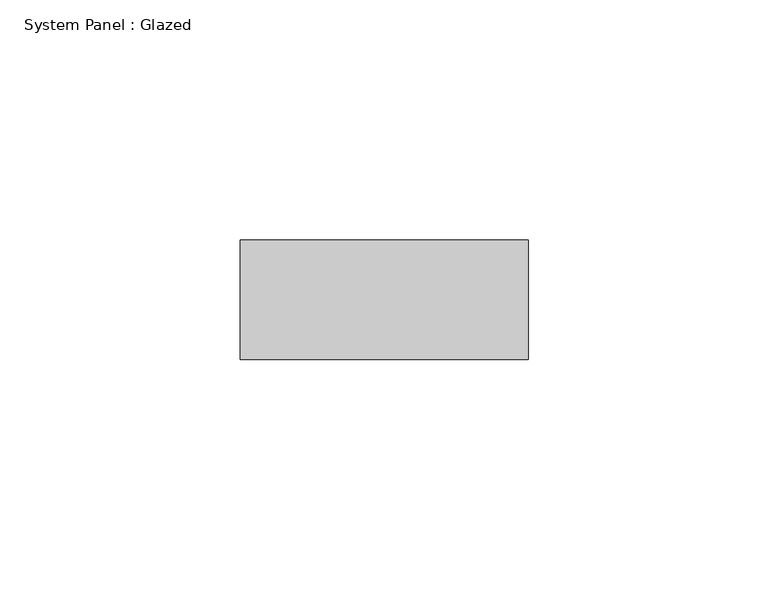
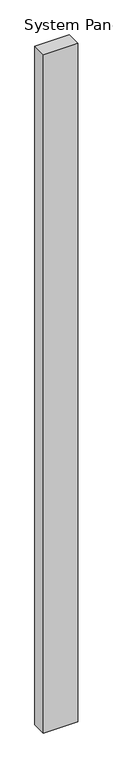
"""IFC4 building model written with IfcOpenShell, lengths in millimetres: plate geometry, System Panel : Glazed."""

from ifc_helpers import new_model, si_unit, origin, origin_with_axes, place, context, project, spatial, polyline, outline, extrude, source, transform, mapped, element, save


def system_panel_glazed_f1160c57(model_context):
    return source(origin(), model_context, "Body", "SweptSolid", [
        extrude(outline(polyline([(30.0, 24.5), (-30.0, 24.5), (-30.0, 49.5), (30.0, 49.5), (30.0, 24.5)])), origin_with_axes(), (0.0, 0.0, 1.0), 1250.0),
    ])


if __name__ == "__main__":
    model = new_model("IFC4")
    model_context = context("Model", 3, world=origin())
    ifc_project = project(units=[si_unit("LENGTHUNIT", "METRE", prefix="MILLI")], contexts=[model_context])
    site = spatial("IfcSite", under=ifc_project)
    building = spatial("IfcBuilding", under=site)
    placement = place(None, origin())
    system_panel_glazed_shape = system_panel_glazed_f1160c57(model_context)
    element("IfcPlate", 1, ObjectType="System Panel : Glazed", at=placement, inside=building, context=model_context, shape_type="MappedRepresentation", body=[
        mapped(system_panel_glazed_shape, transform((0.0, 0.0, 0.0), x_axis=(1.0, 0.0, 0.0), y_axis=(0.0, 1.0, 0.0), z_axis=(0.0, 0.0, 1.0))),
    ])
    save(model, "model.ifc")

# Revit data of these elements
# Element 1 (IfcPlate, "System Panel : Glazed")
#   Materials on its faces: "Glass"
# Materials
#   "Glass": class "Glass", colour RGB 218 227 224, transparency 0.85, Description = "Soda Lime Glass", Cost = 0
